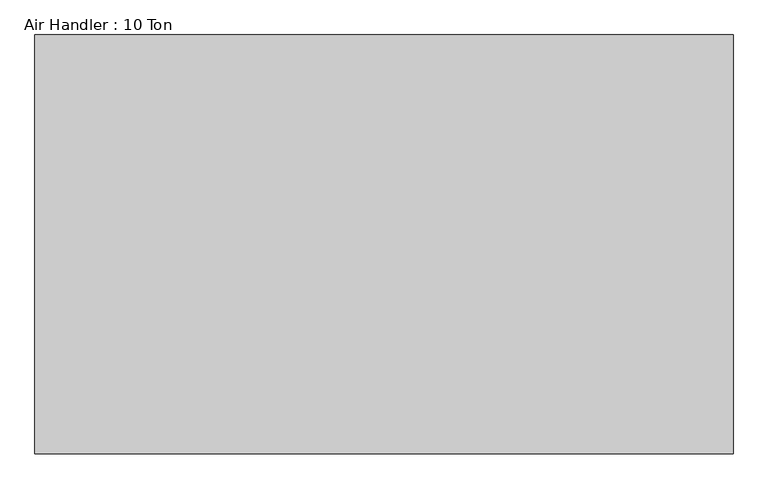
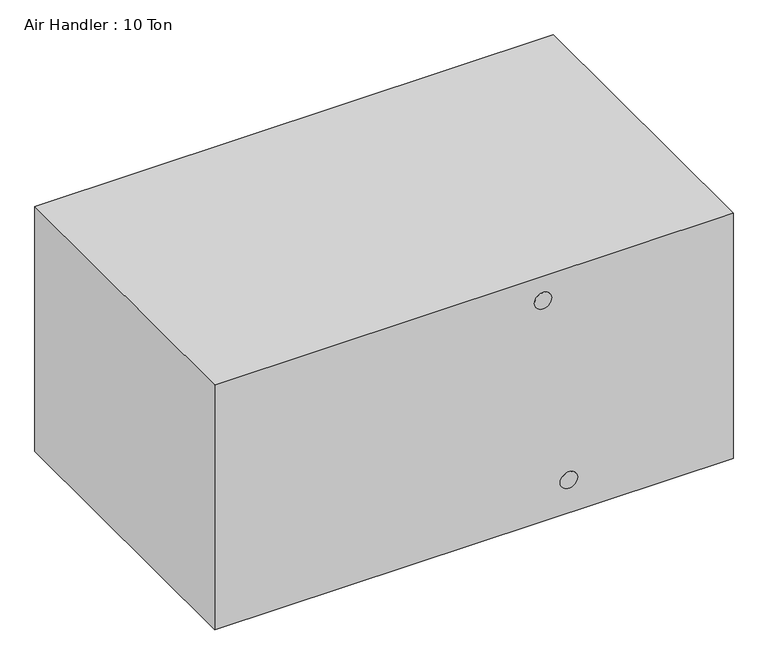
"""IFC4 building model written with IfcOpenShell, lengths in millimetres: proxy geometry, Air Handler : 10 Ton."""

from ifc_helpers import new_model, si_unit, point, frame, frame_2d, origin, origin_with_axes, place, context, project, spatial, polyline, circle_curve, trimmed, segment, composite_curve, outline, extrude, source, transform, mapped, element, save


def air_handler_10_ton_c50fa258(model_context):
    return source(origin(), model_context, "Body", "SweptSolid", [
        extrude(outline(composite_curve([segment(trimmed(circle_curve(frame_2d((1371.6, -1291.43125)), 50.8), [point((1371.6, -1342.23125))], [point((1371.6, -1240.63125))], False, "CARTESIAN"), True, "CONTINUOUS"), segment(trimmed(circle_curve(frame_2d((1371.6, -1291.43125)), 50.8), [point((1371.6, -1240.63125))], [point((1371.6, -1342.23125))], False, "CARTESIAN"), True, "CONTINUOUS")], self_intersect=False)), frame((0.0, -213.9289612, 0.0), z_axis=(0.0, 1.0, 0.0), x_axis=(0.0, 0.0, 1.0)), (0.0, 0.0, 1.0), 26.6039612),
        extrude(outline(composite_curve([segment(trimmed(circle_curve(frame_2d((203.2, -1139.03125)), 50.8), [point((203.2, -1189.83125))], [point((203.2, -1088.23125))], False, "CARTESIAN"), True, "CONTINUOUS"), segment(trimmed(circle_curve(frame_2d((203.2, -1139.03125)), 50.8), [point((203.2, -1088.23125))], [point((203.2, -1189.83125))], False, "CARTESIAN"), True, "CONTINUOUS")], self_intersect=False)), frame((0.0, -213.9289612, 0.0), z_axis=(0.0, 1.0, 0.0), x_axis=(0.0, 0.0, 1.0)), (0.0, 0.0, 1.0), 26.6039612),
        extrude(outline(polyline([(-3221.83125, -213.9289612), (-3221.83125, 1614.8710388), (-173.83125, 1614.8710388), (-173.83125, -213.9289612), (-3221.83125, -213.9289612)])), origin_with_axes(), (0.0, 0.0, 1.0), 1524.0),
    ])


if __name__ == "__main__":
    model = new_model("IFC4")
    model_context = context("Model", 3, world=origin())
    ifc_project = project(units=[si_unit("LENGTHUNIT", "METRE", prefix="MILLI")], contexts=[model_context])
    site = spatial("IfcSite", under=ifc_project)
    building = spatial("IfcBuilding", under=site)
    placement = place(None, origin())
    air_handler_10_ton_shape = air_handler_10_ton_c50fa258(model_context)
    element("IfcBuildingElementProxy", 1, Name="Air Handler : 10 Ton", ObjectType="Air Handler : 10 Ton", at=placement, inside=building, context=model_context, shape_type="MappedRepresentation", body=[
        mapped(air_handler_10_ton_shape, transform((0.0, 0.0, 0.0), x_axis=(1.0, 0.0, 0.0), y_axis=(0.0, 1.0, 0.0), z_axis=(0.0, 0.0, 1.0))),
    ])
    save(model, "model.ifc")

# Revit data of these elements
# Type "Air Handler : 10 Ton"
#   PartShape = "Rectangular Duct"
#   Water Flow [instance default] = 0 GPM
#   Unit Length = 10' - 0"
#   Unit Height = 5' - 0"
#   Unit Width = 6' - 0"
#   Supply Duct Width = 24"
#   Supply Duct Height = 24"
#   Static Pressure Drop [instance default] = 0.00 in-wg
#   ReturnAirFlow [instance default] = 0 CFM
#   IntakeAirFlow [instance default] = 0 CFM
#   Return Duct Width = 42"
#   Return Duct Height = 22"
#   Pipe Radius = 2"
#   Offset - Supply Pipe = 3' - 6"
#   Offset - Supply = 8' - 6"
#   Offset - Return Pipe = 3' - 0"
#   Offset - Return Duct Bottom = 2' - 4"
#   Offset - Return = 1' - 2"
#   Offset - Intake = 5' - 0"
#   Offset - Exhaust = 3' - 0"
#   Intake Height = 1' - 0"
#   Intake Width = 3' - 0"
#   Half Unit Width = 3' - 0"
#   Half Unit Lenght = 5' - 0"
#   ExhaustAirFlow [instance default] = 0 CFM
#   Exhaust Width = 3' - 0"
#   Exhaust Height = 1' - 0"
#   Air Flow [instance default] = 0 CFM
#   Phase = 3
#   Model = ""
#   Assembly Code = ""
# Element 1 (IfcBuildingElementProxy, "Air Handler : 10 Ton")
#   Water Flow = 300 GPM
#   Static Pressure Drop = 1.36 in-wg
#   ReturnAirFlow = 2700 CFM
#   IntakeAirFlow = 962 CFM
#   ExhaustAirFlow = 950 CFM
#   Air Flow = 6355 CFM
